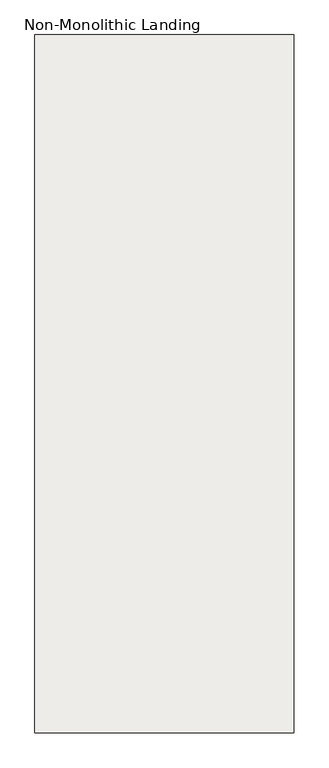
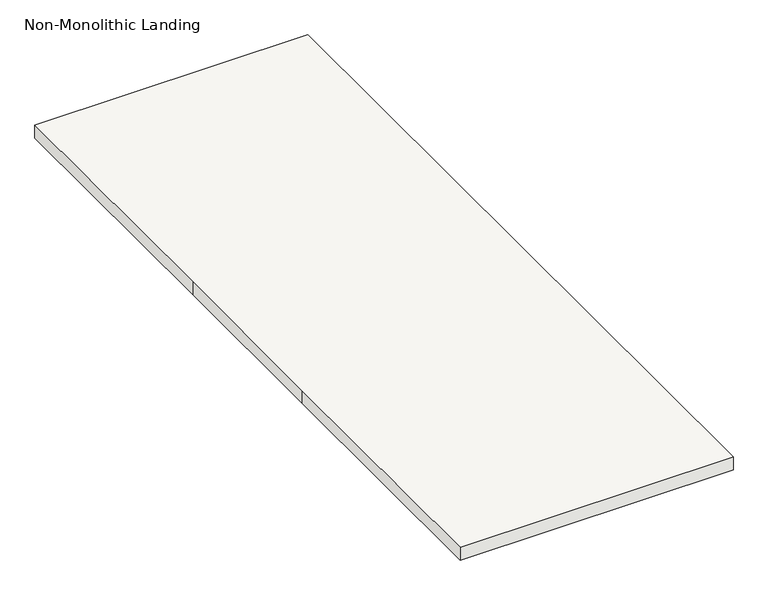
"""IFC4 building model written with IfcOpenShell, lengths in millimetres: slab geometry, Non-Monolithic Landing."""

from ifc_helpers import new_model, si_unit, frame, origin, place, context, project, spatial, polyline, outline, extrude, source, transform, mapped, element, save


def non_monolithic_landing_2b43b373(model_context):
    return source(origin(), model_context, "Body", "SweptSolid", [
        extrude(outline(polyline([(30313.0737371, -705.6098174), (30313.0737371, -9.4804712), (30313.0737371, 990.5195288), (31313.0737371, 990.5195288), (31313.0737371, -1705.6098174), (30313.0737371, -1705.6098174), (30313.0737371, -705.6098174)])), frame((0.0, 0.0, 1714.7058824), z_axis=(0.0, 0.0, 1.0), x_axis=(1.0, 0.0, 0.0)), (0.0, 0.0, 1.0), 50.0),
    ])


if __name__ == "__main__":
    model = new_model("IFC4")
    model_context = context("Model", 3, world=origin())
    ifc_project = project(units=[si_unit("LENGTHUNIT", "METRE", prefix="MILLI")], contexts=[model_context])
    site = spatial("IfcSite", under=ifc_project)
    building = spatial("IfcBuilding", under=site)
    placement = place(None, origin())
    non_monolithic_landing_shape = non_monolithic_landing_2b43b373(model_context)
    element("IfcSlab", 1, ObjectType="Non-Monolithic Landing", at=placement, inside=building, context=model_context, shape_type="MappedRepresentation", body=[
        mapped(non_monolithic_landing_shape, transform((0.0, 0.0, 0.0), x_axis=(1.0, 0.0, 0.0), y_axis=(0.0, 1.0, 0.0), z_axis=(0.0, 0.0, 1.0))),
    ])
    save(model, "model.ifc")
